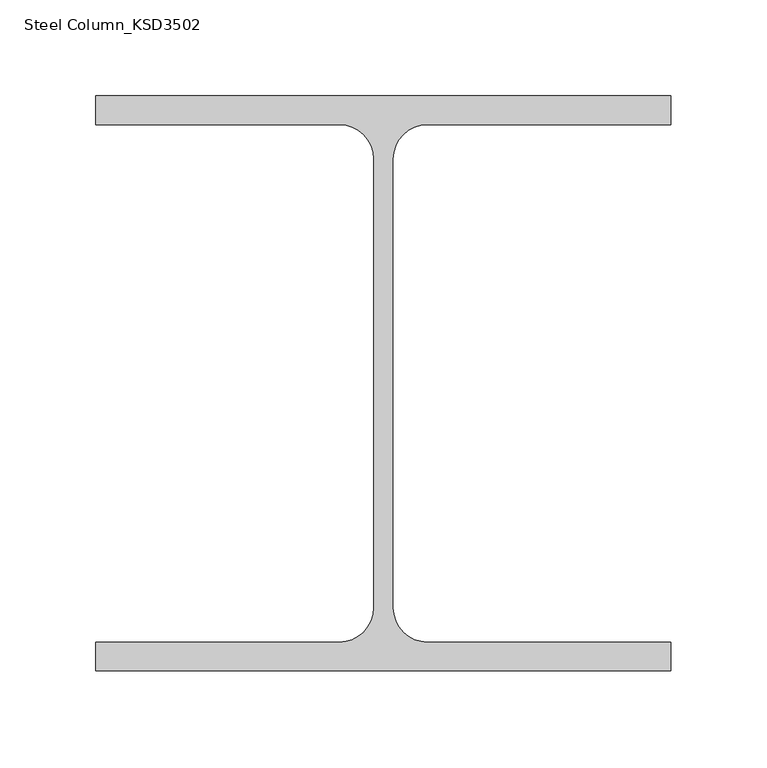
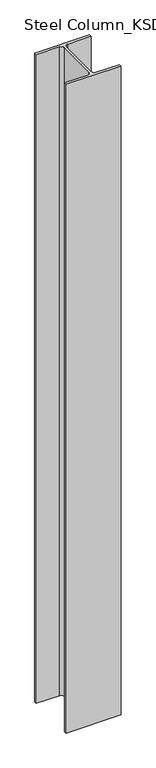
"""IFC4 building model written with IfcOpenShell, lengths in millimetres: column geometry, Steel Column_KSD3502 : H_SC_ASC_H-300×300x10x15."""

from ifc_helpers import new_model, si_unit, point, frame, frame_2d, origin, place, context, project, spatial, polyline, circle_curve, trimmed, segment, composite_curve, outline, extrude, source, transform, mapped, element, save


def steel_column_ksd3502_2bf4f364(model_context):
    return source(origin(), model_context, "Body", "SweptSolid", [
        extrude(outline(composite_curve([segment(polyline([(150.0, 150.0), (150.0, 135.0), (23.0, 135.0)]), True, "CONTINUOUS"), segment(trimmed(circle_curve(frame_2d((23.0, 117.0)), 18.0), [point((23.0, 135.0))], [point((5.0, 117.0))], True, "CARTESIAN"), True, "CONTINUOUS"), segment(polyline([(5.0, 117.0), (5.0, -117.0)]), True, "CONTINUOUS"), segment(trimmed(circle_curve(frame_2d((23.0, -117.0)), 18.0), [point((5.0, -117.0))], [point((23.0, -135.0))], True, "CARTESIAN"), True, "CONTINUOUS"), segment(polyline([(23.0, -135.0), (150.0, -135.0), (150.0, -150.0), (-150.0, -150.0), (-150.0, -135.0), (-23.0, -135.0)]), True, "CONTINUOUS"), segment(trimmed(circle_curve(frame_2d((-23.0, -117.0)), 18.0), [point((-23.0, -135.0))], [point((-5.0, -117.0))], True, "CARTESIAN"), True, "CONTINUOUS"), segment(polyline([(-5.0, -117.0), (-5.0, 117.0)]), True, "CONTINUOUS"), segment(trimmed(circle_curve(frame_2d((-23.0, 117.0)), 18.0), [point((-5.0, 117.0))], [point((-23.0, 135.0))], True, "CARTESIAN"), True, "CONTINUOUS"), segment(polyline([(-23.0, 135.0), (-150.0, 135.0), (-150.0, 150.0), (150.0, 150.0)]), True, "CONTINUOUS")], self_intersect=False)), frame((0.0, 0.0, 685.9720055), z_axis=(0.0, 0.0, 1.0), x_axis=(1.0, 0.0, 0.0)), (0.0, 0.0, 1.0), 3764.0),
    ])


if __name__ == "__main__":
    model = new_model("IFC4")
    model_context = context("Model", 3, world=origin())
    ifc_project = project(units=[si_unit("LENGTHUNIT", "METRE", prefix="MILLI")], contexts=[model_context])
    site = spatial("IfcSite", under=ifc_project)
    building = spatial("IfcBuilding", under=site)
    placement = place(None, origin())
    steel_column_ksd3502_shape = steel_column_ksd3502_2bf4f364(model_context)
    element("IfcColumn", 1, ObjectType="Steel Column_KSD3502 : H_SC_ASC_H-300×300x10x15", at=placement, inside=building, context=model_context, shape_type="MappedRepresentation", body=[
        mapped(steel_column_ksd3502_shape, transform((0.0, 0.0, 0.0), x_axis=(1.0, 0.0, 0.0), y_axis=(0.0, 1.0, 0.0), z_axis=(0.0, 0.0, 1.0))),
    ])
    save(model, "model.ifc")

# Revit data of these elements
# Type "Steel Column_KSD3502 : H_SC_ASC_H-300×300x10x15"
#   Width = 30.0 cm
#   Web Thickness = 1.0 cm
#   Web Fillet = 1.8 cm
#   Warping Constant = 1370670.0 cm⁶
#   Torsional Moment of Inertia = 77.00 cm⁴
#   Section Area = 119.8 cm²
#   Plastic Modulus weak axis = 684.0 cm³
#   Plastic Modulus strong axis = 1500.0 cm³
#   Perimeter = 1.27 m²/m
#   Nominal Weight = 94.00 kgf/m
#   Moment of Inertia weak axis = 6750.00 cm⁴
#   Moment of Inertia strong axis = 20400.00 cm⁴
#   Height = 30.0 cm
#   Flange Thickness = 1.5 cm
#   Elastic Modulus weak axis = 450.0 cm³
#   Elastic Modulus strong axis = 1360.0 cm³
#   Centroid Vertical = 15.0 cm
#   Centroid Horizontal = 15.0 cm
#   Bolt Spacing = 13.97 cm
#   Structural Material [instance default] = Steel, 45-345
#   Section Name Key = ""
#   Assembly Code = ""
# Element 1 (IfcColumn, "Steel Column_KSD3502 : H_SC_ASC_H-300×300x10x15")
#   Structural Material = none
# Materials
#   "Steel, 45-345": class "Metal", colour RGB 189 187 185, transparency 0, Description = "Steel 345 MPa", Cost = 0
